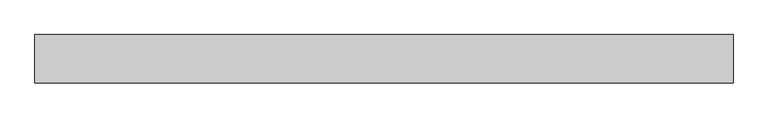
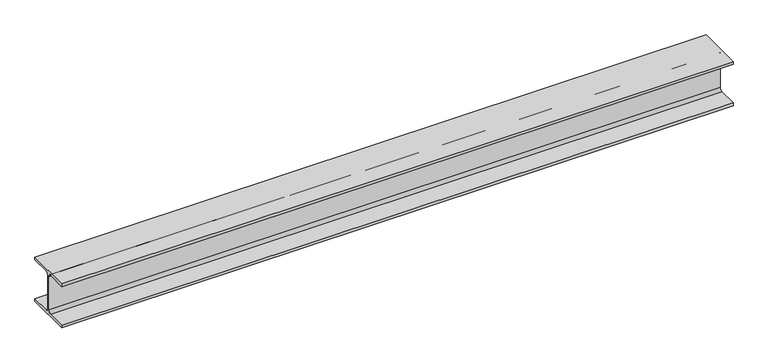
"""IFC4 building model written with IfcOpenShell, lengths in millimetres: beam geometry, 0912_Steel Framing_H-KSD3502 : H_SB_ASB_H-200x200x8x12."""

from ifc_helpers import new_model, si_unit, point, frame, frame_2d, origin, place, context, project, spatial, polyline, circle_curve, trimmed, segment, composite_curve, outline, extrude, source, transform, mapped, element, save


def beam_95991752(model_context):
    return source(origin(), model_context, "Body", "SweptSolid", [
        extrude(outline(composite_curve([segment(polyline([(100.0, -88.0), (100.0, -100.0), (-100.0, -100.0), (-100.0, -88.0), (-17.0, -88.0)]), True, "CONTINUOUS"), segment(trimmed(circle_curve(frame_2d((-17.0, -75.0)), 13.0), [point((-17.0, -88.0))], [point((-4.0, -75.0))], True, "CARTESIAN"), True, "CONTINUOUS"), segment(polyline([(-4.0, -75.0), (-4.0, 75.0)]), True, "CONTINUOUS"), segment(trimmed(circle_curve(frame_2d((-17.0, 75.0)), 13.0), [point((-4.0, 75.0))], [point((-17.0, 88.0))], True, "CARTESIAN"), True, "CONTINUOUS"), segment(polyline([(-17.0, 88.0), (-100.0, 88.0), (-100.0, 100.0), (100.0, 100.0), (100.0, 88.0), (17.0, 88.0)]), True, "CONTINUOUS"), segment(trimmed(circle_curve(frame_2d((17.0, 75.0)), 13.0), [point((17.0, 88.0))], [point((4.0, 75.0))], True, "CARTESIAN"), True, "CONTINUOUS"), segment(polyline([(4.0, 75.0), (4.0, -75.0)]), True, "CONTINUOUS"), segment(trimmed(circle_curve(frame_2d((17.0, -75.0)), 13.0), [point((4.0, -75.0))], [point((17.0, -88.0))], True, "CARTESIAN"), True, "CONTINUOUS"), segment(polyline([(17.0, -88.0), (100.0, -88.0)]), True, "CONTINUOUS")], self_intersect=False)), frame((-1280.1145599, 0.0, 0.0), z_axis=(1.0, 0.0, 0.0), x_axis=(0.0, 1.0, 0.0)), (0.0, 0.0, 1.0), 2889.1530748),
    ])


if __name__ == "__main__":
    model = new_model("IFC4")
    model_context = context("Model", 3, world=origin())
    ifc_project = project(units=[si_unit("LENGTHUNIT", "METRE", prefix="MILLI")], contexts=[model_context])
    site = spatial("IfcSite", under=ifc_project)
    building = spatial("IfcBuilding", under=site)
    placement = place(None, origin())
    beam_shape = beam_95991752(model_context)
    element("IfcBeam", 1, ObjectType="0912_Steel Framing_H-KSD3502 : H_SB_ASB_H-200x200x8x12", at=placement, inside=building, context=model_context, shape_type="MappedRepresentation", body=[
        mapped(beam_shape, transform((0.0, 0.0, 0.0), x_axis=(1.0, 0.0, 0.0), y_axis=(0.0, 1.0, 0.0), z_axis=(0.0, 0.0, 1.0))),
    ])
    save(model, "model.ifc")

# Revit data of these elements
# Type "0912_Steel Framing_H-KSD3502 : H_SB_ASB_H-200x200x8x12"
#   H_WM Code_1 = "S01AA002-00001 | Main Steel Structure Fabrication Work | Shelter/Building | Medium Steel - Standard (90KG/M>Weight≥30KG/M) | Material: (   )"
#   H_WM Code_2 = "S03AA028-00001 | Main Steel Structure Erection Work | Shelter/Building | Medium Steel (90KG/M>Weight≥30KG/M) | Material: (   )"
#   H_WM Code_3 = "S01AA010-00001 | Main Steel Structure Fabrication Work | Shelter/Building | Steel Painting/Coating | for Non-Fireproofed Steel Surface, Surface Preparation, Primer, Second & Final Coat | Material: (   )"
#   H_Q'ty Cal Type Tag = "SB-Q2"
#   Width = 20.0 cm
#   Web Thickness = 0.8 cm
#   Web Fillet = 1.3 cm
#   Warping Constant = 141000.0 cm⁶
#   W = 0
#   Torsional Moment of Inertia = 26.2485 cm⁴
#   Section Area = 63.53 cm²
#   Plastic Modulus weak axis = 244.0 cm³
#   Plastic Modulus strong axis = 525.0 cm³
#   Perimeter = 1.16 m²/m
#   Nominal Weight = 49.90 kgf/m
#   Moment of Inertia weak axis = 1600.00 cm⁴
#   Moment of Inertia strong axis = 4720.00 cm⁴
#   Height = 20.0 cm
#   Flange Thickness = 1.2 cm
#   Elastic Modulus weak axis = 160.0 cm³
#   Elastic Modulus strong axis = 472.0 cm³
#   Centroid Vertical = 10.0 cm
#   Centroid Horizontal = 10.0 cm
#   Ix = 47200000
#   Length [instance default] = 1.5240 m
#   Zx = 525000
#   b = 0.2000 m
#   h = 0.2000 m
#   r = 0.0130 m
#   s = 0.0080 m
#   t = 0.0120 m
#   A = 0.006353 m²
#   Structural Material [instance default] = Steel, 45-345
#   Assembly Code = ""
# Element 1 (IfcBeam, "0912_Steel Framing_H-KSD3502 : H_SB_ASB_H-200x200x8x12")
#   Structural Material = none
# Materials
#   "Steel, 45-345": class "Metal", colour RGB 189 187 185, transparency 0, Description = "Steel 345 MPa", Cost = 0
